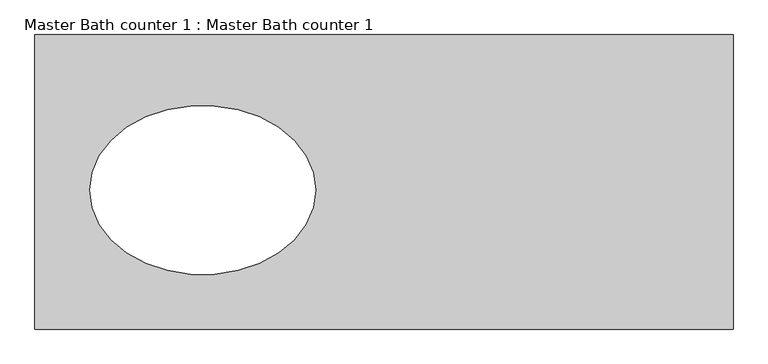
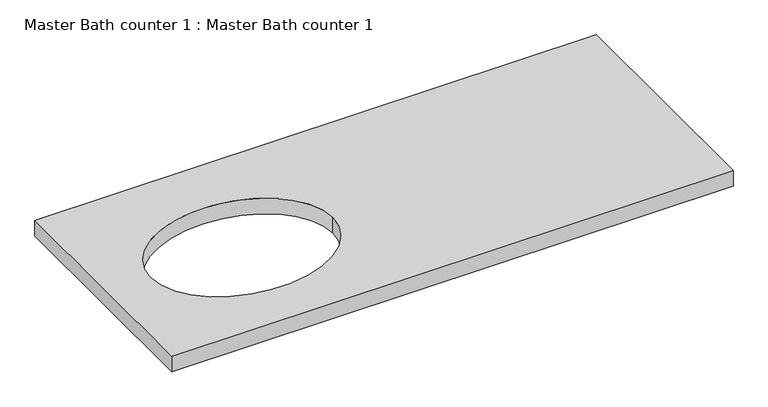
"""IFC4 building model written with IfcOpenShell, lengths in millimetres: furniture geometry, Master Bath counter 1 : Master Bath counter 1."""

from ifc_helpers import new_model, si_unit, point, frame, origin, place, context, project, spatial, ellipse_curve, trimmed, source, transform, mapped, element, save
from ifc_brep_helpers import plane_surface, extruded_surface, advanced_brep


def master_bath_counter_1_master_bath_counter_1_0aba8c7c(model_context):
    return source(origin(), model_context, "Body", "AdvancedBrep", [
        advanced_brep(
        [(-7255.2952631, 15722.6, 800.1), (-7255.2952631, 15170.15, 800.1), (-8564.5625, 15170.15, 800.1), (-8564.5625, 15722.6, 800.1), (-8038.1062701, 15431.1837135, 800.1), (-8462.1062701, 15431.1837135, 800.1), (-7255.2952631, 15722.6, 838.2), (-8564.5625, 15722.6, 838.2), (-8564.5625, 15170.15, 838.2), (-7255.2952631, 15170.15, 838.2), (-8038.1062701, 15431.1837135, 838.2), (-8462.1062701, 15431.1837135, 838.2)],
        [
            (0, 1),
            (1, 2),
            (2, 3),
            (3, 0),
            (4, 5, ellipse_curve(frame((-8250.1062701, 15431.1837135, 800.1), z_axis=(0.0, 0.0, 1.0), x_axis=(-1.0, 0.0, 0.0)), 212.0, 158.7697221)),
            (5, 4, ellipse_curve(frame((-8250.1062701, 15431.1837135, 800.1), z_axis=(0.0, 0.0, 1.0), x_axis=(-1.0, 0.0, 0.0)), 212.0, 158.7697221)),
            (6, 7),
            (7, 8),
            (8, 9),
            (9, 6),
            (10, 11, ellipse_curve(frame((-8250.1062701, 15431.1837135, 838.2), z_axis=(0.0, 0.0, -1.0), x_axis=(-1.0, 0.0, 0.0)), 212.0, 158.7697221)),
            (11, 10, ellipse_curve(frame((-8250.1062701, 15431.1837135, 838.2), z_axis=(0.0, 0.0, -1.0), x_axis=(-1.0, 0.0, 0.0)), 212.0, 158.7697221)),
            (6, 0),
            (3, 7),
            (2, 8),
            (1, 9),
            (10, 4),
            (5, 11),
        ],
        [
            plane_surface(frame((-8564.5625, 15722.6, 800.1), z_axis=(0.0, 0.0, -1.0), x_axis=(1.0, 0.0, 0.0))),
            plane_surface(frame((-8564.5625, 15722.6, 838.2), z_axis=(0.0, 0.0, 1.0), x_axis=(-1.0, 0.0, 0.0))),
            plane_surface(frame((-7255.2952631, 15722.6, 838.2), z_axis=(0.0, 1.0, 0.0), x_axis=(0.0, 0.0, -1.0))),
            plane_surface(frame((-8564.5625, 15722.6, 838.2), z_axis=(-1.0, 0.0, 0.0), x_axis=(0.0, 0.0, -1.0))),
            plane_surface(frame((-8564.5625, 15170.15, 838.2), z_axis=(0.0, -1.0, 0.0), x_axis=(0.0, 0.0, -1.0))),
            plane_surface(frame((-7255.2952631, 15170.15, 838.2), z_axis=(1.0, 0.0, 0.0), x_axis=(0.0, 0.0, -1.0))),
            extruded_surface(trimmed(ellipse_curve(frame((-8250.1062701, 15431.1837135, -38.1), z_axis=(0.0, 0.0, -1.0), x_axis=(-1.0, 0.0, 0.0)), 212.0, 158.7697221), [point((-8038.1062701, 15431.1837135, -38.1))], [point((-8462.1062701, 15431.1837135, -38.1))], True, "CARTESIAN"), (0.0, 0.0, 38.1), 38.1),
            extruded_surface(trimmed(ellipse_curve(frame((-8250.1062701, 15431.1837135, -38.1), z_axis=(0.0, 0.0, -1.0), x_axis=(-1.0, 0.0, 0.0)), 212.0, 158.7697221), [point((-8462.1062701, 15431.1837135, -38.1))], [point((-8038.1062701, 15431.1837135, -38.1))], True, "CARTESIAN"), (0.0, 0.0, 38.1), 38.1),
        ],
        [
            (0, [[1, 2, 3, 4], [5, 6]]),
            (1, [[7, 8, 9, 10], [11, 12]]),
            (2, [[-7, 13, -4, 14]]),
            (3, [[-8, -14, -3, 15]]),
            (4, [[-9, -15, -2, 16]]),
            (5, [[-10, -16, -1, -13]]),
            (6, [[-11, 17, -6, 18]]),
            (7, [[-12, -18, -5, -17]]),
        ],
    ),
    ])


if __name__ == "__main__":
    model = new_model("IFC4")
    model_context = context("Model", 3, world=origin())
    ifc_project = project(units=[si_unit("LENGTHUNIT", "METRE", prefix="MILLI")], contexts=[model_context])
    site = spatial("IfcSite", under=ifc_project)
    building = spatial("IfcBuilding", under=site)
    placement = place(None, origin())
    master_bath_counter_1_master_bath_counter_1_shape = master_bath_counter_1_master_bath_counter_1_0aba8c7c(model_context)
    element("IfcFurniture", 1, ObjectType="Master Bath counter 1 : Master Bath counter 1", at=placement, inside=building, context=model_context, shape_type="MappedRepresentation", body=[
        mapped(master_bath_counter_1_master_bath_counter_1_shape, transform((0.0, 0.0, 0.0), x_axis=(1.0, 0.0, 0.0), y_axis=(0.0, 1.0, 0.0), z_axis=(0.0, 0.0, 1.0))),
    ])
    save(model, "model.ifc")

# Revit data of these elements
# Type "Master Bath counter 1 : Master Bath counter 1"
#   COBie.Type = no
# Element 1 (IfcFurniture, "Master Bath counter 1 : Master Bath counter 1")
#   Materials on its faces: "Corian - Emerald"
# Materials
#   "Corian - Emerald": class "Plastic", colour RGB 51 95 44, transparency 0, Cost = 0
